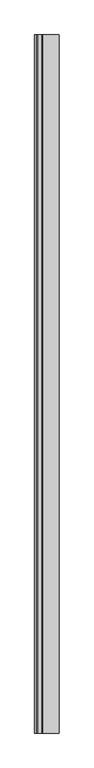
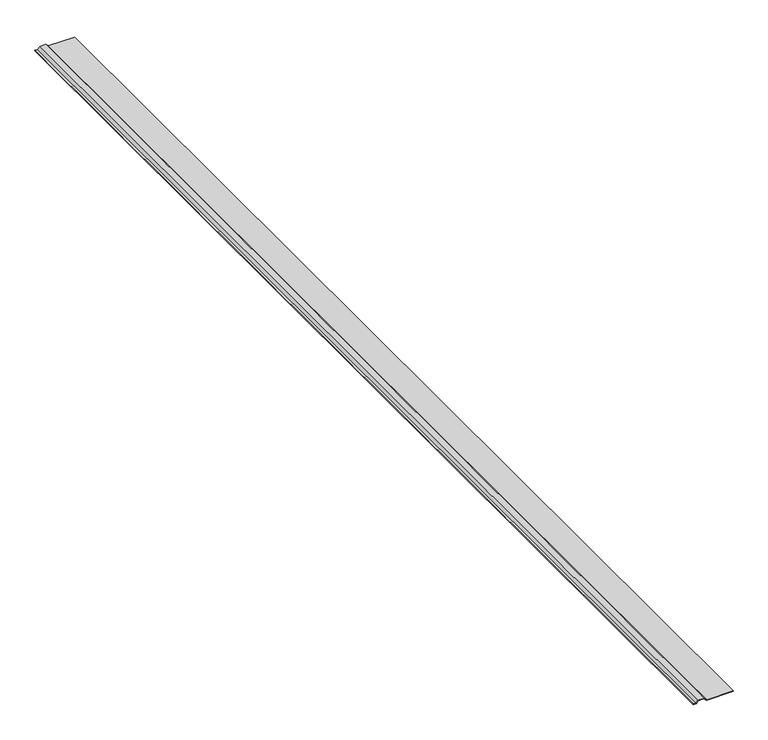
"""IFC4 building model written with IfcOpenShell, lengths in millimetres: proxy geometry, BEND PANEL2:BEND PANEL005:297554 : BEND PANEL2:BEND PANEL005:297554."""

from ifc_helpers import new_model, si_unit, point, frame, frame_2d, origin, place, context, project, spatial, polyline, circle_curve, trimmed, segment, composite_curve, outline, extrude, source, transform, mapped, element, save


def generic_models_d3e8673c(model_context):
    return source(origin(), model_context, "Body", "SweptSolid", [
        extrude(outline(composite_curve([segment(polyline([(42575.4212949, 10625.7246965), (42575.4212949, 10672.2321774), (42576.61192, 10672.2321774), (42576.61192, 10625.7246965), (42580.7948047, 10621.5418118), (42580.7948047, 10610.5733587), (42576.61192, 10606.390474), (42576.61192, 10602.5174326), (42575.4212949, 10602.5174326), (42575.4212949, 10606.390474)]), True, "CONTINUOUS"), segment(trimmed(circle_curve(frame_2d((42576.6119199, 10606.390474)), 1.190625), [point((42575.4212949, 10606.390474))], [point((42575.7700209, 10607.232373))], False, "CARTESIAN"), True, "CONTINUOUS"), segment(polyline([(42575.7700209, 10607.232373), (42579.6041796, 10611.0665317), (42579.6041796, 10621.0486388), (42575.7700209, 10624.8827975)]), True, "CONTINUOUS"), segment(trimmed(circle_curve(frame_2d((42576.6119199, 10625.7246965)), 1.190625), [point((42575.7700209, 10624.8827975))], [point((42575.4212949, 10625.7246965))], False, "CARTESIAN"), True, "CONTINUOUS")], self_intersect=False)), frame((0.0, -774.5581163, 0.0), z_axis=(0.0, 1.0, 0.0), x_axis=(0.0, 0.0, 1.0)), (0.0, 0.0, 1.0), 1999.85),
    ])


if __name__ == "__main__":
    model = new_model("IFC4")
    model_context = context("Model", 3, world=origin())
    ifc_project = project(units=[si_unit("LENGTHUNIT", "METRE", prefix="MILLI")], contexts=[model_context])
    site = spatial("IfcSite", under=ifc_project)
    building = spatial("IfcBuilding", under=site)
    placement = place(None, origin())
    generic_models_shape = generic_models_d3e8673c(model_context)
    element("IfcBuildingElementProxy", 1, Name="BEND PANEL2:BEND PANEL005:297554 : BEND PANEL2:BEND PANEL005:297554", ObjectType="BEND PANEL2:BEND PANEL005:297554 : BEND PANEL2:BEND PANEL005:297554", at=placement, inside=building, context=model_context, shape_type="MappedRepresentation", body=[
        mapped(generic_models_shape, transform((0.0, 0.0, 0.0), x_axis=(1.0, 0.0, 0.0), y_axis=(0.0, 1.0, 0.0), z_axis=(0.0, 0.0, 1.0))),
    ])
    save(model, "model.ifc")

# Revit data of these elements
# Type "BEND PANEL2:BEND PANEL005:297554 : BEND PANEL2:BEND PANEL005:297554"
#   NameOverride = "BEND PANEL2:BEND PANEL005:297554"
#   ObjectTypeOverride = "BEND PANEL2:BEND PANEL005"
#   Reference = "BEND PANEL005"
#   Category = "Generic Models"
#   Tag = "297554"
# Element 1 (IfcBuildingElementProxy, "BEND PANEL2:BEND PANEL005:297554 : BEND PANEL2:BEND PANEL005:297554")
#   Materials on its faces: "METAL PROFILE"
# Materials
#   "METAL PROFILE": class "Unassigned", colour RGB 128 128 128, transparency 0
